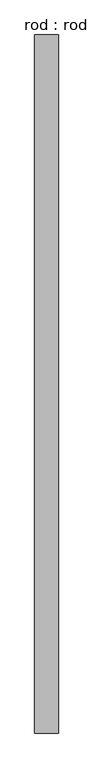
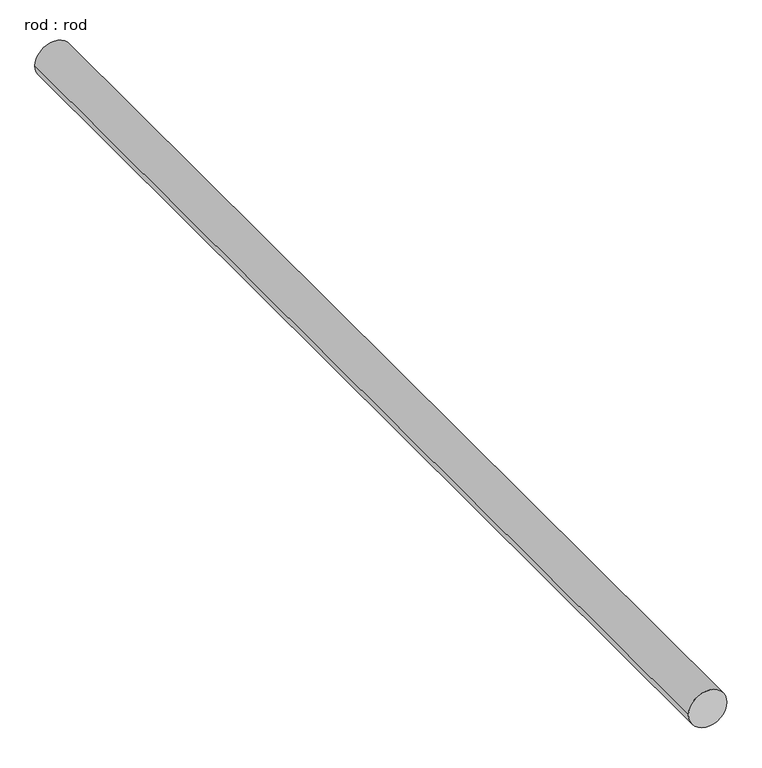
"""IFC4 building model written with IfcOpenShell, lengths in millimetres: proxy geometry, rod : rod."""

from ifc_helpers import new_model, si_unit, point, frame, frame_2d, origin, place, context, project, spatial, circle_curve, trimmed, segment, composite_curve, outline, extrude, source, transform, mapped, element, save


def rod_rod_9080f142(model_context):
    return source(origin(), model_context, "Body", "SweptSolid", [
        extrude(outline(composite_curve([segment(trimmed(circle_curve(frame_2d((0.0108462, 0.0)), 200.0), [point((0.0108462, 200.0))], [point((0.0108462, -200.0))], False, "CARTESIAN"), True, "CONTINUOUS"), segment(trimmed(circle_curve(frame_2d((0.0108462, 0.0)), 200.0), [point((0.0108462, -200.0))], [point((0.0108462, 200.0))], False, "CARTESIAN"), True, "CONTINUOUS")], self_intersect=False)), frame((0.0, -1820.0641958, 0.0), z_axis=(0.0, 1.0, 0.0), x_axis=(0.0, 0.0, 1.0)), (0.0, 0.0, 1.0), 11825.5856222),
    ])


if __name__ == "__main__":
    model = new_model("IFC4")
    model_context = context("Model", 3, world=origin())
    ifc_project = project(units=[si_unit("LENGTHUNIT", "METRE", prefix="MILLI")], contexts=[model_context])
    site = spatial("IfcSite", under=ifc_project)
    building = spatial("IfcBuilding", under=site)
    placement = place(None, origin())
    rod_rod_shape = rod_rod_9080f142(model_context)
    element("IfcBuildingElementProxy", 1, Name="rod : rod", ObjectType="rod : rod", at=placement, inside=building, context=model_context, shape_type="MappedRepresentation", body=[
        mapped(rod_rod_shape, transform((0.0, 0.0, 0.0), x_axis=(1.0, 0.0, 0.0), y_axis=(0.0, 1.0, 0.0), z_axis=(0.0, 0.0, 1.0))),
    ])
    save(model, "model.ifc")

# Revit data of these elements
# Type "rod : rod"
#   Default Elevation = 0
